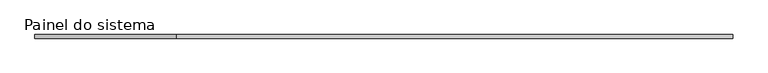
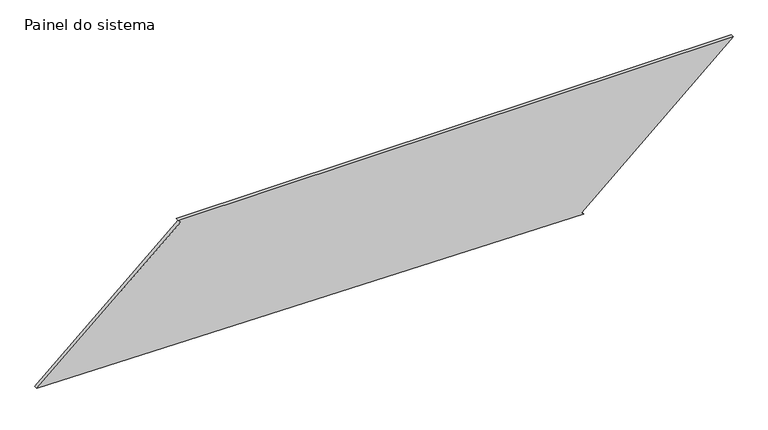
"""IFC4 building model written with IfcOpenShell, lengths in millimetres: plate geometry, Painel do sistema : Envidraçado."""

import ifcopenshell
import ifcopenshell.guid

model = None  # the IFC model being written
_history = None  # IfcOwnerHistory: only IFC2X3 demands one
_inside = {}  # id of a spatial element -> (the spatial element, [elements in it])
_under = {}  # id of a project, library or spatial element -> (it, [spatial elements below it])
_declared = {}  # id of a project -> (the project, [libraries it declares])
_typed = {}  # id of a type object -> (the type object, [elements of that type])
_made_of = {}  # id of a material, layer set ... -> (it, [elements and type objects made of it])


def new_model(schema):
    """Start an empty IFC model of exactly this schema.

    Asked for "IFC4X3", IfcOpenShell would pick the latest addendum, in which some entities
    have other attributes; the version numbers below select the first issue.
    IFC2X3 requires an IfcOwnerHistory on every rooted entity: one is made here for all.
    """
    global model, _history
    if schema == "IFC4X3":
        model = ifcopenshell.file(schema_version=(4, 3, 0, 0))
    else:
        model = ifcopenshell.file(schema=schema)
    _inside.clear()
    _under.clear()
    _declared.clear()
    _typed.clear()
    _made_of.clear()
    _history = None
    if model.schema == "IFC2X3":
        org = make("IfcOrganization", Name="unknown")
        user = make(
            "IfcPersonAndOrganization",
            ThePerson=make("IfcPerson", FamilyName="unknown"),
            TheOrganization=org,
        )
        app = make(
            "IfcApplication",
            ApplicationDeveloper=org,
            Version="unknown",
            ApplicationFullName="unknown",
            ApplicationIdentifier="unknown",
        )
        _history = make(
            "IfcOwnerHistory",
            OwningUser=user,
            OwningApplication=app,
            ChangeAction="ADDED",
            CreationDate=0,
        )
    return model


def make(cls, **values):
    """One entity of the class cls with the attributes given. An attribute that is None is left unset."""
    return model.create_entity(
        cls, **{name: value for name, value in values.items() if value is not None}
    )


def rooted(cls, **values):
    """An entity with a GlobalId (a new one), such as an element, a storey or a relation."""
    return make(cls, GlobalId=ifcopenshell.guid.new(), OwnerHistory=_history, **values)


def si_unit(unit_type, name, prefix=None):
    """IfcSIUnit, for example si_unit("LENGTHUNIT", "METRE", prefix="MILLI")."""
    return make("IfcSIUnit", UnitType=unit_type, Prefix=prefix, Name=name)


def assignment(units):
    """IfcUnitAssignment: the units of a project."""
    return None if units is None else make("IfcUnitAssignment", Units=units)


def point(xyz):
    """IfcCartesianPoint."""
    return None if xyz is None else make("IfcCartesianPoint", Coordinates=xyz)


def direction(xyz):
    """IfcDirection."""
    return None if xyz is None else make("IfcDirection", DirectionRatios=xyz)


def frame(location, z_axis=None, x_axis=None):
    """IfcAxis2Placement3D, a coordinate frame: its origin and axes. An axis left out is left unset."""
    return make(
        "IfcAxis2Placement3D",
        Location=point(location),
        Axis=direction(z_axis),
        RefDirection=direction(x_axis),
    )


def origin():
    """The frame at (0, 0, 0) with its axes left unset."""
    return frame((0.0, 0.0, 0.0))


def place(relative_to, where):
    """IfcLocalPlacement: puts the frame where relative to a parent placement (None: the world)."""
    return make(
        "IfcLocalPlacement", PlacementRelTo=relative_to, RelativePlacement=where
    )


def context(
    kind, dimensions, precision=None, world=None, true_north=None, identifier=None
):
    """IfcGeometricRepresentationContext, for example the 3D "Model" context."""
    return make(
        "IfcGeometricRepresentationContext",
        ContextIdentifier=identifier,
        ContextType=kind,
        CoordinateSpaceDimension=dimensions,
        Precision=precision,
        WorldCoordinateSystem=world,
        TrueNorth=true_north,
    )


def project(units=None, contexts=None):
    """IfcProject with its units and contexts."""
    return rooted(
        "IfcProject",
        Name="project",
        RepresentationContexts=contexts,
        UnitsInContext=assignment(units),
    )


def spatial(cls, under=None, at=None, **own):
    """A site, building, storey or space (cls), placed at a placement, below another one or the project."""
    s = rooted(cls, ObjectPlacement=at, **own)
    if under is not None:
        _under.setdefault(under.id(), (under, []))[1].append(s)
    return s


def polyline(points):
    """IfcPolyline through the points."""
    return make("IfcPolyline", Points=[point(p) for p in points])


def outline(outer, holes=None, kind="AREA"):
    """IfcArbitraryClosedProfileDef: a profile drawn as a closed curve; with holes, ...WithVoids."""
    if holes is None:
        return make("IfcArbitraryClosedProfileDef", ProfileType=kind, OuterCurve=outer)
    return make(
        "IfcArbitraryProfileDefWithVoids",
        ProfileType=kind,
        OuterCurve=outer,
        InnerCurves=holes,
    )


def extrude(swept, where, along, depth):
    """IfcExtrudedAreaSolid: the profile swept, set in the frame where, extruded along a direction by depth."""
    return make(
        "IfcExtrudedAreaSolid",
        SweptArea=swept,
        Position=where,
        ExtrudedDirection=direction(along),
        Depth=depth,
    )


def shape(context_of_items, identifier, shape_type, items):
    """IfcShapeRepresentation: the items that make up one representation, for example the "Body"."""
    return make(
        "IfcShapeRepresentation",
        ContextOfItems=context_of_items,
        RepresentationIdentifier=identifier,
        RepresentationType=shape_type,
        Items=items,
    )


def source(mapping_origin, context_of_items, identifier, shape_type, items):
    """IfcRepresentationMap: a shape defined once, which mapped items show again and again."""
    return make(
        "IfcRepresentationMap",
        MappingOrigin=mapping_origin,
        MappedRepresentation=shape(context_of_items, identifier, shape_type, items),
    )


def transform(
    local_origin,
    x_axis=None,
    y_axis=None,
    z_axis=None,
    scale=None,
    scale2=None,
    scale3=None,
    uniform=True,
):
    """IfcCartesianTransformationOperator3D, or its non-uniform kind. x_axis, y_axis, z_axis: its Axis1, 2, 3."""
    if uniform:
        return make(
            "IfcCartesianTransformationOperator3D",
            Axis1=direction(x_axis),
            Axis2=direction(y_axis),
            LocalOrigin=point(local_origin),
            Scale=scale,
            Axis3=direction(z_axis),
        )
    return make(
        "IfcCartesianTransformationOperator3DnonUniform",
        Axis1=direction(x_axis),
        Axis2=direction(y_axis),
        LocalOrigin=point(local_origin),
        Scale=scale,
        Axis3=direction(z_axis),
        Scale2=scale2,
        Scale3=scale3,
    )


def mapped(mapping_source, mapping_target):
    """IfcMappedItem: shows the shape of a source again, moved by a transform."""
    return make(
        "IfcMappedItem", MappingSource=mapping_source, MappingTarget=mapping_target
    )


def made_of(thing, what):
    """Note that an element or type object is made of a material, layer set ...; save() writes the relation."""
    if what is not None:
        _made_of.setdefault(what.id(), (what, []))[1].append(thing)
    return thing


def element(
    cls,
    number,
    at=None,
    inside=None,
    cuts=None,
    type_object=None,
    material=None,
    context=None,
    identifier="Body",
    shape_type=None,
    held_by="IfcProductDefinitionShape",
    body=None,
    shapes=None,
    **own,
):
    """One element of the class cls, such as IfcWall. Its Tag is "e" and its number.

    at: its placement. inside: the storey or other place that contains it. cuts: it is an
    opening in that element (IfcRelVoidsElement). A single representation is given by context,
    identifier, shape_type and body (its items); several are given by shapes. held_by: the class
    of the entity that holds the representations. save() writes the other relations.
    """
    e = rooted(cls, Tag="e%d" % number, ObjectPlacement=at, **own)
    if body is not None:
        shapes = [shape(context, identifier, shape_type, body)]
    if shapes is not None:
        e.Representation = make(held_by, Representations=shapes)
    if inside is not None:
        _inside.setdefault(inside.id(), (inside, []))[1].append(e)
    if cuts is not None:
        rooted(
            "IfcRelVoidsElement", RelatingBuildingElement=cuts, RelatedOpeningElement=e
        )
    if type_object is not None:
        _typed.setdefault(type_object.id(), (type_object, []))[1].append(e)
    return made_of(e, material)


def aggregate(whole, parts):
    """IfcRelAggregates: a whole, such as a stair, and the parts it consists of."""
    return rooted("IfcRelAggregates", RelatingObject=whole, RelatedObjects=parts)


def save(model, path):
    """Write the relations noted so far, then the file.

    IfcRelAggregates (storeys below a building ...), IfcRelContainedInSpatialStructure (elements
    in a storey), IfcRelDefinesByType, IfcRelAssociatesMaterial and IfcRelDeclares: one each for
    every whole, place, type object, material and project.
    """
    for whole, parts in _under.values():
        aggregate(whole, parts)
    for where, things in _inside.values():
        rooted(
            "IfcRelContainedInSpatialStructure",
            RelatedElements=things,
            RelatingStructure=where,
        )
    for kind, things in _typed.values():
        rooted("IfcRelDefinesByType", RelatedObjects=things, RelatingType=kind)
    for what, things in _made_of.values():
        rooted("IfcRelAssociatesMaterial", RelatedObjects=things, RelatingMaterial=what)
    for by, libraries in _declared.values():
        rooted("IfcRelDeclares", RelatingContext=by, RelatedDefinitions=libraries)
    model.write(path)


def painel_do_sistema_9628f676(model_context):
    return source(origin(), model_context, "Body", "SweptSolid", [
        extrude(outline(polyline([(0.0, 1386.1710796), (18.8079041, 1369.7010237), (943.3782695, 2425.5098731), (943.3782695, -1441.551887), (924.5703654, -1425.0818311), (48.4968973, -2425.5098731), (0.0, 1386.1710796)])), frame((0.0, 24.5, 0.0), z_axis=(0.0, 1.0, 0.0), x_axis=(0.0, 0.0, 1.0)), (0.0, 0.0, 1.0), 25.0),
    ])


if __name__ == "__main__":
    model = new_model("IFC4")
    model_context = context("Model", 3, world=origin())
    ifc_project = project(units=[si_unit("LENGTHUNIT", "METRE", prefix="MILLI")], contexts=[model_context])
    site = spatial("IfcSite", under=ifc_project)
    building = spatial("IfcBuilding", under=site)
    placement = place(None, origin())
    painel_do_sistema_shape = painel_do_sistema_9628f676(model_context)
    element("IfcPlate", 1, ObjectType="Painel do sistema : Envidraçado", at=placement, inside=building, context=model_context, shape_type="MappedRepresentation", body=[
        mapped(painel_do_sistema_shape, transform((0.0, 0.0, 0.0), x_axis=(1.0, 0.0, 0.0), y_axis=(0.0, 1.0, 0.0), z_axis=(0.0, 0.0, 1.0))),
    ])
    save(model, "model.ifc")

# Revit data of these elements
# Type "Painel do sistema : Envidraçado"
#   Construction Type Id = "GSP4R"
#   Analytic Construction = "Vidraça única Pilkington 1/8 pol"
#   Visual Light Transmittance = 0.9
#   Solar Heat Gain Coefficient = 0.86
#   Heat Transfer Coefficient (U) = 6.7069 W/(m²·K)
# Element 1 (IfcPlate, "Painel do sistema : Envidraçado")
#   Materials on its faces: "Vidro"
# Materials
#   "Vidro": class "Vidro", colour RGB 0 128 192, transparency 0.9, Description = "Vidro de sílica", Cost = 0
